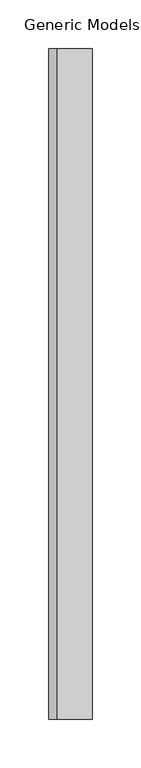
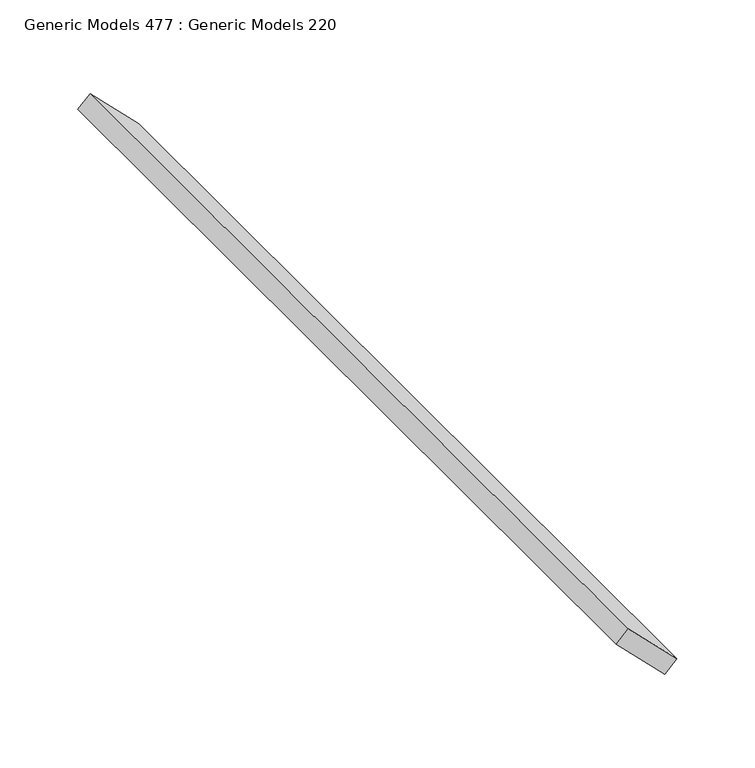
"""IFC4 building model written with IfcOpenShell, lengths in millimetres: proxy geometry, Generic Models 477 : Generic Models 220."""

from ifc_helpers import new_model, si_unit, frame, origin, place, context, project, spatial, polyline, outline, extrude, source, transform, mapped, element, save


def generic_models_477_generic_models_220_0972c5b9(model_context):
    return source(origin(), model_context, "Body", "SweptSolid", [
        extrude(outline(polyline([(0.0, -50.8), (0.0, 0.0), (690.8142348, 0.0), (690.8142348, -50.8), (0.0, -50.8)])), frame((-6899.085451, -4564.8872686, 127942.1762561), z_axis=(0.7071067811865582, 0.0, 0.7071067811865369), x_axis=(0.0, 1.0, 0.0)), (0.0, 0.0, 1.0), 12.7),
    ])


if __name__ == "__main__":
    model = new_model("IFC4")
    model_context = context("Model", 3, world=origin())
    ifc_project = project(units=[si_unit("LENGTHUNIT", "METRE", prefix="MILLI")], contexts=[model_context])
    site = spatial("IfcSite", under=ifc_project)
    building = spatial("IfcBuilding", under=site)
    placement = place(None, origin())
    generic_models_477_generic_models_220_shape = generic_models_477_generic_models_220_0972c5b9(model_context)
    element("IfcBuildingElementProxy", 1, Name="Generic Models 477 : Generic Models 220", ObjectType="Generic Models 477 : Generic Models 220", at=placement, inside=building, context=model_context, shape_type="MappedRepresentation", body=[
        mapped(generic_models_477_generic_models_220_shape, transform((0.0, 0.0, 0.0), x_axis=(1.0, 0.0, 0.0), y_axis=(0.0, 1.0, 0.0), z_axis=(0.0, 0.0, 1.0))),
    ])
    save(model, "model.ifc")

# Revit data of these elements
# Element 1 (IfcBuildingElementProxy, "Generic Models 477 : Generic Models 220")
#   Materials on its faces: "_WOOD TONE ALUMINUM EXTRUSION SLAT BY KNOTWOOD"
# Materials
#   "_WOOD TONE ALUMINUM EXTRUSION SLAT BY KNOTWOOD": class "Generic", colour RGB 177 130 114, transparency 0, Cost = 0
